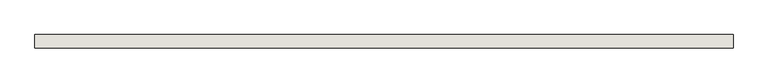
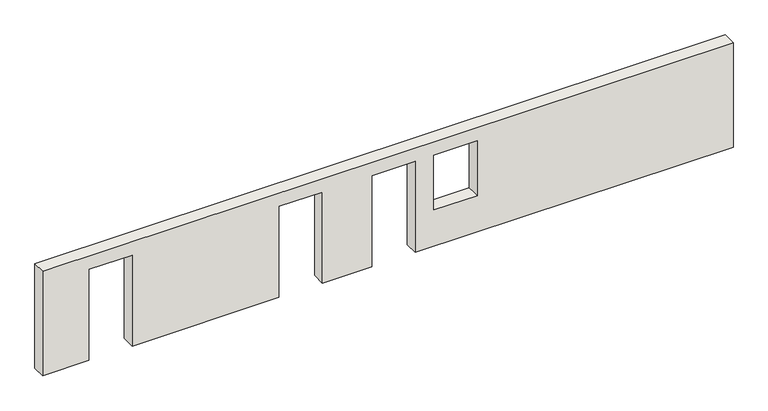
"""IFC4 building model written with IfcOpenShell, lengths in millimetres: wall geometry, 0_3d_modell."""

import ifcopenshell
import ifcopenshell.guid

model = None  # the IFC model being written
_history = None  # IfcOwnerHistory: only IFC2X3 demands one
_inside = {}  # id of a spatial element -> (the spatial element, [elements in it])
_under = {}  # id of a project, library or spatial element -> (it, [spatial elements below it])
_declared = {}  # id of a project -> (the project, [libraries it declares])
_typed = {}  # id of a type object -> (the type object, [elements of that type])
_made_of = {}  # id of a material, layer set ... -> (it, [elements and type objects made of it])


def new_model(schema):
    """Start an empty IFC model of exactly this schema.

    Asked for "IFC4X3", IfcOpenShell would pick the latest addendum, in which some entities
    have other attributes; the version numbers below select the first issue.
    IFC2X3 requires an IfcOwnerHistory on every rooted entity: one is made here for all.
    """
    global model, _history
    if schema == "IFC4X3":
        model = ifcopenshell.file(schema_version=(4, 3, 0, 0))
    else:
        model = ifcopenshell.file(schema=schema)
    _inside.clear()
    _under.clear()
    _declared.clear()
    _typed.clear()
    _made_of.clear()
    _history = None
    if model.schema == "IFC2X3":
        org = make("IfcOrganization", Name="unknown")
        user = make(
            "IfcPersonAndOrganization",
            ThePerson=make("IfcPerson", FamilyName="unknown"),
            TheOrganization=org,
        )
        app = make(
            "IfcApplication",
            ApplicationDeveloper=org,
            Version="unknown",
            ApplicationFullName="unknown",
            ApplicationIdentifier="unknown",
        )
        _history = make(
            "IfcOwnerHistory",
            OwningUser=user,
            OwningApplication=app,
            ChangeAction="ADDED",
            CreationDate=0,
        )
    return model


def make(cls, **values):
    """One entity of the class cls with the attributes given. An attribute that is None is left unset."""
    return model.create_entity(
        cls, **{name: value for name, value in values.items() if value is not None}
    )


def rooted(cls, **values):
    """An entity with a GlobalId (a new one), such as an element, a storey or a relation."""
    return make(cls, GlobalId=ifcopenshell.guid.new(), OwnerHistory=_history, **values)


def si_unit(unit_type, name, prefix=None):
    """IfcSIUnit, for example si_unit("LENGTHUNIT", "METRE", prefix="MILLI")."""
    return make("IfcSIUnit", UnitType=unit_type, Prefix=prefix, Name=name)


def assignment(units):
    """IfcUnitAssignment: the units of a project."""
    return None if units is None else make("IfcUnitAssignment", Units=units)


def point(xyz):
    """IfcCartesianPoint."""
    return None if xyz is None else make("IfcCartesianPoint", Coordinates=xyz)


def direction(xyz):
    """IfcDirection."""
    return None if xyz is None else make("IfcDirection", DirectionRatios=xyz)


def frame(location, z_axis=None, x_axis=None):
    """IfcAxis2Placement3D, a coordinate frame: its origin and axes. An axis left out is left unset."""
    return make(
        "IfcAxis2Placement3D",
        Location=point(location),
        Axis=direction(z_axis),
        RefDirection=direction(x_axis),
    )


def origin():
    """The frame at (0, 0, 0) with its axes left unset."""
    return frame((0.0, 0.0, 0.0))


def place(relative_to, where):
    """IfcLocalPlacement: puts the frame where relative to a parent placement (None: the world)."""
    return make(
        "IfcLocalPlacement", PlacementRelTo=relative_to, RelativePlacement=where
    )


def context(
    kind, dimensions, precision=None, world=None, true_north=None, identifier=None
):
    """IfcGeometricRepresentationContext, for example the 3D "Model" context."""
    return make(
        "IfcGeometricRepresentationContext",
        ContextIdentifier=identifier,
        ContextType=kind,
        CoordinateSpaceDimension=dimensions,
        Precision=precision,
        WorldCoordinateSystem=world,
        TrueNorth=true_north,
    )


def project(units=None, contexts=None):
    """IfcProject with its units and contexts."""
    return rooted(
        "IfcProject",
        Name="project",
        RepresentationContexts=contexts,
        UnitsInContext=assignment(units),
    )


def spatial(cls, under=None, at=None, **own):
    """A site, building, storey or space (cls), placed at a placement, below another one or the project."""
    s = rooted(cls, ObjectPlacement=at, **own)
    if under is not None:
        _under.setdefault(under.id(), (under, []))[1].append(s)
    return s


def polyline(points):
    """IfcPolyline through the points."""
    return make("IfcPolyline", Points=[point(p) for p in points])


def outline(outer, holes=None, kind="AREA"):
    """IfcArbitraryClosedProfileDef: a profile drawn as a closed curve; with holes, ...WithVoids."""
    if holes is None:
        return make("IfcArbitraryClosedProfileDef", ProfileType=kind, OuterCurve=outer)
    return make(
        "IfcArbitraryProfileDefWithVoids",
        ProfileType=kind,
        OuterCurve=outer,
        InnerCurves=holes,
    )


def extrude(swept, where, along, depth):
    """IfcExtrudedAreaSolid: the profile swept, set in the frame where, extruded along a direction by depth."""
    return make(
        "IfcExtrudedAreaSolid",
        SweptArea=swept,
        Position=where,
        ExtrudedDirection=direction(along),
        Depth=depth,
    )


def shape(context_of_items, identifier, shape_type, items):
    """IfcShapeRepresentation: the items that make up one representation, for example the "Body"."""
    return make(
        "IfcShapeRepresentation",
        ContextOfItems=context_of_items,
        RepresentationIdentifier=identifier,
        RepresentationType=shape_type,
        Items=items,
    )


def source(mapping_origin, context_of_items, identifier, shape_type, items):
    """IfcRepresentationMap: a shape defined once, which mapped items show again and again."""
    return make(
        "IfcRepresentationMap",
        MappingOrigin=mapping_origin,
        MappedRepresentation=shape(context_of_items, identifier, shape_type, items),
    )


def transform(
    local_origin,
    x_axis=None,
    y_axis=None,
    z_axis=None,
    scale=None,
    scale2=None,
    scale3=None,
    uniform=True,
):
    """IfcCartesianTransformationOperator3D, or its non-uniform kind. x_axis, y_axis, z_axis: its Axis1, 2, 3."""
    if uniform:
        return make(
            "IfcCartesianTransformationOperator3D",
            Axis1=direction(x_axis),
            Axis2=direction(y_axis),
            LocalOrigin=point(local_origin),
            Scale=scale,
            Axis3=direction(z_axis),
        )
    return make(
        "IfcCartesianTransformationOperator3DnonUniform",
        Axis1=direction(x_axis),
        Axis2=direction(y_axis),
        LocalOrigin=point(local_origin),
        Scale=scale,
        Axis3=direction(z_axis),
        Scale2=scale2,
        Scale3=scale3,
    )


def mapped(mapping_source, mapping_target):
    """IfcMappedItem: shows the shape of a source again, moved by a transform."""
    return make(
        "IfcMappedItem", MappingSource=mapping_source, MappingTarget=mapping_target
    )


def made_of(thing, what):
    """Note that an element or type object is made of a material, layer set ...; save() writes the relation."""
    if what is not None:
        _made_of.setdefault(what.id(), (what, []))[1].append(thing)
    return thing


def element(
    cls,
    number,
    at=None,
    inside=None,
    cuts=None,
    type_object=None,
    material=None,
    context=None,
    identifier="Body",
    shape_type=None,
    held_by="IfcProductDefinitionShape",
    body=None,
    shapes=None,
    **own,
):
    """One element of the class cls, such as IfcWall. Its Tag is "e" and its number.

    at: its placement. inside: the storey or other place that contains it. cuts: it is an
    opening in that element (IfcRelVoidsElement). A single representation is given by context,
    identifier, shape_type and body (its items); several are given by shapes. held_by: the class
    of the entity that holds the representations. save() writes the other relations.
    """
    e = rooted(cls, Tag="e%d" % number, ObjectPlacement=at, **own)
    if body is not None:
        shapes = [shape(context, identifier, shape_type, body)]
    if shapes is not None:
        e.Representation = make(held_by, Representations=shapes)
    if inside is not None:
        _inside.setdefault(inside.id(), (inside, []))[1].append(e)
    if cuts is not None:
        rooted(
            "IfcRelVoidsElement", RelatingBuildingElement=cuts, RelatedOpeningElement=e
        )
    if type_object is not None:
        _typed.setdefault(type_object.id(), (type_object, []))[1].append(e)
    return made_of(e, material)


def aggregate(whole, parts):
    """IfcRelAggregates: a whole, such as a stair, and the parts it consists of."""
    return rooted("IfcRelAggregates", RelatingObject=whole, RelatedObjects=parts)


def save(model, path):
    """Write the relations noted so far, then the file.

    IfcRelAggregates (storeys below a building ...), IfcRelContainedInSpatialStructure (elements
    in a storey), IfcRelDefinesByType, IfcRelAssociatesMaterial and IfcRelDeclares: one each for
    every whole, place, type object, material and project.
    """
    for whole, parts in _under.values():
        aggregate(whole, parts)
    for where, things in _inside.values():
        rooted(
            "IfcRelContainedInSpatialStructure",
            RelatedElements=things,
            RelatingStructure=where,
        )
    for kind, things in _typed.values():
        rooted("IfcRelDefinesByType", RelatedObjects=things, RelatingType=kind)
    for what, things in _made_of.values():
        rooted("IfcRelAssociatesMaterial", RelatedObjects=things, RelatingMaterial=what)
    for by, libraries in _declared.values():
        rooted("IfcRelDeclares", RelatingContext=by, RelatedDefinitions=libraries)
    model.write(path)


def wall_f6c49615(model_context):
    return source(origin(), model_context, "Body", "SweptSolid", [
        extrude(outline(polyline([(2510.0, 9709.9644869), (0.0, 9709.9644869), (0.0, 18002.8619019), (2880.0, 18002.8619019), (2880.0, 0.0), (0.0, 0.0), (0.0, 1200.0), (2510.0, 1200.0), (2510.0, 2335.0), (0.0, 2335.0), (0.0, 6160.3619019), (2510.0, 6160.3619019), (2510.0, 7295.3619019), (0.0, 7295.3619019), (0.0, 8574.9644869), (2510.0, 8574.9644869), (2510.0, 9709.9644869)]), holes=[polyline([(2510.0, 11328.4823196), (1000.0, 11328.4823196), (1000.0, 10193.4823196), (2510.0, 10193.4823196), (2510.0, 11328.4823196)])]), frame((0.0, 0.0, 0.0), z_axis=(0.0, 1.0, 0.0), x_axis=(0.0, 0.0, 1.0)), (0.0, 0.0, 1.0), 350.0),
    ])


if __name__ == "__main__":
    model = new_model("IFC4")
    model_context = context("Model", 3, world=origin())
    ifc_project = project(units=[si_unit("LENGTHUNIT", "METRE", prefix="MILLI")], contexts=[model_context])
    site = spatial("IfcSite", under=ifc_project)
    building = spatial("IfcBuilding", under=site)
    placement = place(None, origin())
    wall_shape = wall_f6c49615(model_context)
    element("IfcWall", 1, ObjectType="0_3d_modell", at=placement, inside=building, context=model_context, shape_type="MappedRepresentation", body=[
        mapped(wall_shape, transform((0.0, 0.0, 0.0), x_axis=(1.0, 0.0, 0.0), y_axis=(0.0, 1.0, 0.0), z_axis=(0.0, 0.0, 1.0))),
    ])
    save(model, "model.ifc")

# Revit data of these elements
# Element 1 (IfcWall, "0_3d_modell")
#   Materials on its faces: "holzschalung"
# Materials
#   "holzschalung": class "Unassigned", colour RGB 128 128 128, transparency 0
